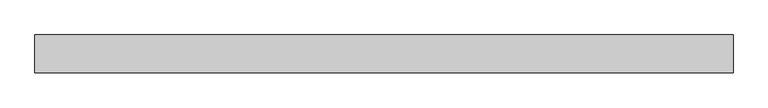
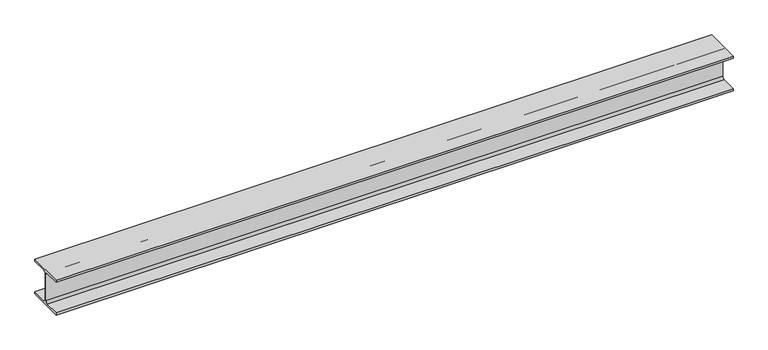
"""IFC4 building model written with IfcOpenShell, lengths in millimetres: beam geometry, 0912_Steel Framing_H-KSD3502 : H_SB_ASB_H-200x200x8x12."""

from ifc_helpers import new_model, si_unit, point, frame, frame_2d, origin, place, context, project, spatial, polyline, circle_curve, trimmed, segment, composite_curve, outline, extrude, source, transform, mapped, element, save


def beam_9ed8c8cf(model_context):
    return source(origin(), model_context, "Body", "SweptSolid", [
        extrude(outline(composite_curve([segment(polyline([(-100.0, -88.0), (-17.0, -88.0)]), True, "CONTINUOUS"), segment(trimmed(circle_curve(frame_2d((-17.0, -75.0)), 13.0), [point((-17.0, -88.0))], [point((-4.0, -75.0))], True, "CARTESIAN"), True, "CONTINUOUS"), segment(polyline([(-4.0, -75.0), (-4.0, 75.0)]), True, "CONTINUOUS"), segment(trimmed(circle_curve(frame_2d((-17.0, 75.0)), 13.0), [point((-4.0, 75.0))], [point((-17.0, 88.0))], True, "CARTESIAN"), True, "CONTINUOUS"), segment(polyline([(-17.0, 88.0), (-100.0, 88.0), (-100.0, 100.0), (100.0, 100.0), (100.0, 88.0), (17.0, 88.0)]), True, "CONTINUOUS"), segment(trimmed(circle_curve(frame_2d((17.0, 75.0)), 13.0), [point((17.0, 88.0))], [point((4.0, 75.0))], True, "CARTESIAN"), True, "CONTINUOUS"), segment(polyline([(4.0, 75.0), (4.0, -75.0)]), True, "CONTINUOUS"), segment(trimmed(circle_curve(frame_2d((17.0, -75.0)), 13.0), [point((4.0, -75.0))], [point((17.0, -88.0))], True, "CARTESIAN"), True, "CONTINUOUS"), segment(polyline([(17.0, -88.0), (100.0, -88.0), (100.0, -100.0), (-100.0, -100.0), (-100.0, -88.0)]), True, "CONTINUOUS")], self_intersect=False)), frame((-1864.7392612, 0.0, 0.0), z_axis=(1.0, 0.0, 0.0), x_axis=(0.0, 1.0, 0.0)), (0.0, 0.0, 1.0), 3677.145122),
    ])


if __name__ == "__main__":
    model = new_model("IFC4")
    model_context = context("Model", 3, world=origin())
    ifc_project = project(units=[si_unit("LENGTHUNIT", "METRE", prefix="MILLI")], contexts=[model_context])
    site = spatial("IfcSite", under=ifc_project)
    building = spatial("IfcBuilding", under=site)
    placement = place(None, origin())
    beam_shape = beam_9ed8c8cf(model_context)
    element("IfcBeam", 1, ObjectType="0912_Steel Framing_H-KSD3502 : H_SB_ASB_H-200x200x8x12", at=placement, inside=building, context=model_context, shape_type="MappedRepresentation", body=[
        mapped(beam_shape, transform((0.0, 0.0, 0.0), x_axis=(1.0, 0.0, 0.0), y_axis=(0.0, 1.0, 0.0), z_axis=(0.0, 0.0, 1.0))),
    ])
    save(model, "model.ifc")

# Revit data of these elements
# Type "0912_Steel Framing_H-KSD3502 : H_SB_ASB_H-200x200x8x12"
#   H_WM Code_1 = "S01AA002-00001 | Main Steel Structure Fabrication Work | Shelter/Building | Medium Steel - Standard (90KG/M>Weight≥30KG/M) | Material: (   )"
#   H_WM Code_2 = "S03AA028-00001 | Main Steel Structure Erection Work | Shelter/Building | Medium Steel (90KG/M>Weight≥30KG/M) | Material: (   )"
#   H_WM Code_3 = "S01AA010-00001 | Main Steel Structure Fabrication Work | Shelter/Building | Steel Painting/Coating | for Non-Fireproofed Steel Surface, Surface Preparation, Primer, Second & Final Coat | Material: (   )"
#   H_Q'ty Cal Type Tag = "SB-Q2"
#   Width = 20.0 cm
#   Web Thickness = 0.8 cm
#   Web Fillet = 1.3 cm
#   Warping Constant = 141000.0 cm⁶
#   W = 0
#   Torsional Moment of Inertia = 26.2485 cm⁴
#   Section Area = 63.53 cm²
#   Plastic Modulus weak axis = 244.0 cm³
#   Plastic Modulus strong axis = 525.0 cm³
#   Perimeter = 1.16 m²/m
#   Nominal Weight = 49.90 kgf/m
#   Moment of Inertia weak axis = 1600.00 cm⁴
#   Moment of Inertia strong axis = 4720.00 cm⁴
#   Height = 20.0 cm
#   Flange Thickness = 1.2 cm
#   Elastic Modulus weak axis = 160.0 cm³
#   Elastic Modulus strong axis = 472.0 cm³
#   Centroid Vertical = 10.0 cm
#   Centroid Horizontal = 10.0 cm
#   Ix = 47200000
#   Length [instance default] = 1.5240 m
#   Zx = 525000
#   b = 0.2000 m
#   h = 0.2000 m
#   r = 0.0130 m
#   s = 0.0080 m
#   t = 0.0120 m
#   A = 0.006353 m²
#   Structural Material [instance default] = Steel, 45-345
#   Assembly Code = ""
# Element 1 (IfcBeam, "0912_Steel Framing_H-KSD3502 : H_SB_ASB_H-200x200x8x12")
#   Structural Material = none
# Materials
#   "Steel, 45-345": class "Metal", colour RGB 189 187 185, transparency 0, Description = "Steel 345 MPa", Cost = 0
